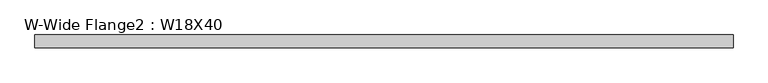
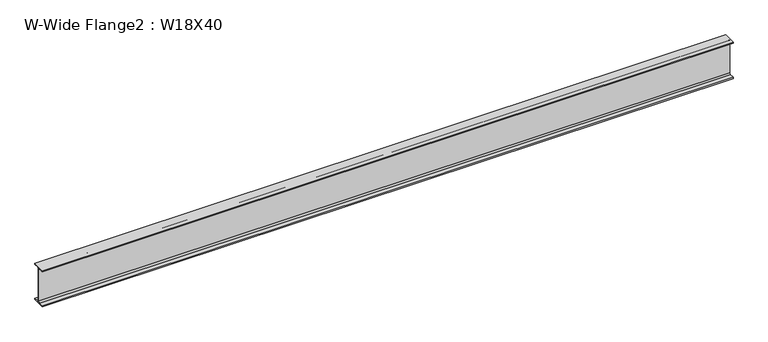
"""IFC4 building model written with IfcOpenShell, lengths in millimetres: beam geometry, W-Wide Flange2 : W18X40."""

import ifcopenshell
import ifcopenshell.guid

model = None  # the IFC model being written
_history = None  # IfcOwnerHistory: only IFC2X3 demands one
_inside = {}  # id of a spatial element -> (the spatial element, [elements in it])
_under = {}  # id of a project, library or spatial element -> (it, [spatial elements below it])
_declared = {}  # id of a project -> (the project, [libraries it declares])
_typed = {}  # id of a type object -> (the type object, [elements of that type])
_made_of = {}  # id of a material, layer set ... -> (it, [elements and type objects made of it])


def new_model(schema):
    """Start an empty IFC model of exactly this schema.

    Asked for "IFC4X3", IfcOpenShell would pick the latest addendum, in which some entities
    have other attributes; the version numbers below select the first issue.
    IFC2X3 requires an IfcOwnerHistory on every rooted entity: one is made here for all.
    """
    global model, _history
    if schema == "IFC4X3":
        model = ifcopenshell.file(schema_version=(4, 3, 0, 0))
    else:
        model = ifcopenshell.file(schema=schema)
    _inside.clear()
    _under.clear()
    _declared.clear()
    _typed.clear()
    _made_of.clear()
    _history = None
    if model.schema == "IFC2X3":
        org = make("IfcOrganization", Name="unknown")
        user = make(
            "IfcPersonAndOrganization",
            ThePerson=make("IfcPerson", FamilyName="unknown"),
            TheOrganization=org,
        )
        app = make(
            "IfcApplication",
            ApplicationDeveloper=org,
            Version="unknown",
            ApplicationFullName="unknown",
            ApplicationIdentifier="unknown",
        )
        _history = make(
            "IfcOwnerHistory",
            OwningUser=user,
            OwningApplication=app,
            ChangeAction="ADDED",
            CreationDate=0,
        )
    return model


def make(cls, **values):
    """One entity of the class cls with the attributes given. An attribute that is None is left unset."""
    return model.create_entity(
        cls, **{name: value for name, value in values.items() if value is not None}
    )


def rooted(cls, **values):
    """An entity with a GlobalId (a new one), such as an element, a storey or a relation."""
    return make(cls, GlobalId=ifcopenshell.guid.new(), OwnerHistory=_history, **values)


def si_unit(unit_type, name, prefix=None):
    """IfcSIUnit, for example si_unit("LENGTHUNIT", "METRE", prefix="MILLI")."""
    return make("IfcSIUnit", UnitType=unit_type, Prefix=prefix, Name=name)


def assignment(units):
    """IfcUnitAssignment: the units of a project."""
    return None if units is None else make("IfcUnitAssignment", Units=units)


def point(xyz):
    """IfcCartesianPoint."""
    return None if xyz is None else make("IfcCartesianPoint", Coordinates=xyz)


def direction(xyz):
    """IfcDirection."""
    return None if xyz is None else make("IfcDirection", DirectionRatios=xyz)


def frame(location, z_axis=None, x_axis=None):
    """IfcAxis2Placement3D, a coordinate frame: its origin and axes. An axis left out is left unset."""
    return make(
        "IfcAxis2Placement3D",
        Location=point(location),
        Axis=direction(z_axis),
        RefDirection=direction(x_axis),
    )


def frame_2d(location, x_axis=None):
    """IfcAxis2Placement2D, a coordinate frame in the plane: its origin and x axis."""
    return make(
        "IfcAxis2Placement2D", Location=point(location), RefDirection=direction(x_axis)
    )


def origin():
    """The frame at (0, 0, 0) with its axes left unset."""
    return frame((0.0, 0.0, 0.0))


def place(relative_to, where):
    """IfcLocalPlacement: puts the frame where relative to a parent placement (None: the world)."""
    return make(
        "IfcLocalPlacement", PlacementRelTo=relative_to, RelativePlacement=where
    )


def context(
    kind, dimensions, precision=None, world=None, true_north=None, identifier=None
):
    """IfcGeometricRepresentationContext, for example the 3D "Model" context."""
    return make(
        "IfcGeometricRepresentationContext",
        ContextIdentifier=identifier,
        ContextType=kind,
        CoordinateSpaceDimension=dimensions,
        Precision=precision,
        WorldCoordinateSystem=world,
        TrueNorth=true_north,
    )


def project(units=None, contexts=None):
    """IfcProject with its units and contexts."""
    return rooted(
        "IfcProject",
        Name="project",
        RepresentationContexts=contexts,
        UnitsInContext=assignment(units),
    )


def spatial(cls, under=None, at=None, **own):
    """A site, building, storey or space (cls), placed at a placement, below another one or the project."""
    s = rooted(cls, ObjectPlacement=at, **own)
    if under is not None:
        _under.setdefault(under.id(), (under, []))[1].append(s)
    return s


def polyline(points):
    """IfcPolyline through the points."""
    return make("IfcPolyline", Points=[point(p) for p in points])


def circle_curve(where, radius):
    """IfcCircle in the frame where."""
    return make("IfcCircle", Position=where, Radius=radius)


def trimmed(basis, trim1, trim2, sense, master):
    """IfcTrimmedCurve: the piece of a basis curve between two trims."""
    return make(
        "IfcTrimmedCurve",
        BasisCurve=basis,
        Trim1=trim1,
        Trim2=trim2,
        SenseAgreement=sense,
        MasterRepresentation=master,
    )


def segment(curve, same_sense, transition):
    """IfcCompositeCurveSegment."""
    return make(
        "IfcCompositeCurveSegment",
        Transition=transition,
        SameSense=same_sense,
        ParentCurve=curve,
    )


def composite_curve(segments, self_intersect=None):
    """IfcCompositeCurve: segments joined end to end."""
    return make("IfcCompositeCurve", Segments=segments, SelfIntersect=self_intersect)


def outline(outer, holes=None, kind="AREA"):
    """IfcArbitraryClosedProfileDef: a profile drawn as a closed curve; with holes, ...WithVoids."""
    if holes is None:
        return make("IfcArbitraryClosedProfileDef", ProfileType=kind, OuterCurve=outer)
    return make(
        "IfcArbitraryProfileDefWithVoids",
        ProfileType=kind,
        OuterCurve=outer,
        InnerCurves=holes,
    )


def extrude(swept, where, along, depth):
    """IfcExtrudedAreaSolid: the profile swept, set in the frame where, extruded along a direction by depth."""
    return make(
        "IfcExtrudedAreaSolid",
        SweptArea=swept,
        Position=where,
        ExtrudedDirection=direction(along),
        Depth=depth,
    )


def shape(context_of_items, identifier, shape_type, items):
    """IfcShapeRepresentation: the items that make up one representation, for example the "Body"."""
    return make(
        "IfcShapeRepresentation",
        ContextOfItems=context_of_items,
        RepresentationIdentifier=identifier,
        RepresentationType=shape_type,
        Items=items,
    )


def source(mapping_origin, context_of_items, identifier, shape_type, items):
    """IfcRepresentationMap: a shape defined once, which mapped items show again and again."""
    return make(
        "IfcRepresentationMap",
        MappingOrigin=mapping_origin,
        MappedRepresentation=shape(context_of_items, identifier, shape_type, items),
    )


def transform(
    local_origin,
    x_axis=None,
    y_axis=None,
    z_axis=None,
    scale=None,
    scale2=None,
    scale3=None,
    uniform=True,
):
    """IfcCartesianTransformationOperator3D, or its non-uniform kind. x_axis, y_axis, z_axis: its Axis1, 2, 3."""
    if uniform:
        return make(
            "IfcCartesianTransformationOperator3D",
            Axis1=direction(x_axis),
            Axis2=direction(y_axis),
            LocalOrigin=point(local_origin),
            Scale=scale,
            Axis3=direction(z_axis),
        )
    return make(
        "IfcCartesianTransformationOperator3DnonUniform",
        Axis1=direction(x_axis),
        Axis2=direction(y_axis),
        LocalOrigin=point(local_origin),
        Scale=scale,
        Axis3=direction(z_axis),
        Scale2=scale2,
        Scale3=scale3,
    )


def mapped(mapping_source, mapping_target):
    """IfcMappedItem: shows the shape of a source again, moved by a transform."""
    return make(
        "IfcMappedItem", MappingSource=mapping_source, MappingTarget=mapping_target
    )


def made_of(thing, what):
    """Note that an element or type object is made of a material, layer set ...; save() writes the relation."""
    if what is not None:
        _made_of.setdefault(what.id(), (what, []))[1].append(thing)
    return thing


def element(
    cls,
    number,
    at=None,
    inside=None,
    cuts=None,
    type_object=None,
    material=None,
    context=None,
    identifier="Body",
    shape_type=None,
    held_by="IfcProductDefinitionShape",
    body=None,
    shapes=None,
    **own,
):
    """One element of the class cls, such as IfcWall. Its Tag is "e" and its number.

    at: its placement. inside: the storey or other place that contains it. cuts: it is an
    opening in that element (IfcRelVoidsElement). A single representation is given by context,
    identifier, shape_type and body (its items); several are given by shapes. held_by: the class
    of the entity that holds the representations. save() writes the other relations.
    """
    e = rooted(cls, Tag="e%d" % number, ObjectPlacement=at, **own)
    if body is not None:
        shapes = [shape(context, identifier, shape_type, body)]
    if shapes is not None:
        e.Representation = make(held_by, Representations=shapes)
    if inside is not None:
        _inside.setdefault(inside.id(), (inside, []))[1].append(e)
    if cuts is not None:
        rooted(
            "IfcRelVoidsElement", RelatingBuildingElement=cuts, RelatedOpeningElement=e
        )
    if type_object is not None:
        _typed.setdefault(type_object.id(), (type_object, []))[1].append(e)
    return made_of(e, material)


def aggregate(whole, parts):
    """IfcRelAggregates: a whole, such as a stair, and the parts it consists of."""
    return rooted("IfcRelAggregates", RelatingObject=whole, RelatedObjects=parts)


def save(model, path):
    """Write the relations noted so far, then the file.

    IfcRelAggregates (storeys below a building ...), IfcRelContainedInSpatialStructure (elements
    in a storey), IfcRelDefinesByType, IfcRelAssociatesMaterial and IfcRelDeclares: one each for
    every whole, place, type object, material and project.
    """
    for whole, parts in _under.values():
        aggregate(whole, parts)
    for where, things in _inside.values():
        rooted(
            "IfcRelContainedInSpatialStructure",
            RelatedElements=things,
            RelatingStructure=where,
        )
    for kind, things in _typed.values():
        rooted("IfcRelDefinesByType", RelatedObjects=things, RelatingType=kind)
    for what, things in _made_of.values():
        rooted("IfcRelAssociatesMaterial", RelatedObjects=things, RelatingMaterial=what)
    for by, libraries in _declared.values():
        rooted("IfcRelDeclares", RelatingContext=by, RelatedDefinitions=libraries)
    model.write(path)


def w_wide_flange2_w18x40_2ea4b68e(model_context):
    return source(origin(), model_context, "Body", "SweptSolid", [
        extrude(outline(composite_curve([segment(polyline([(76.454, -213.995), (76.454, -227.33), (-76.454, -227.33), (-76.454, -213.995), (-20.828, -213.995)]), True, "CONTINUOUS"), segment(trimmed(circle_curve(frame_2d((-20.828, -197.1675)), 16.8275), [point((-20.828, -213.995))], [point((-4.0005, -197.1675))], True, "CARTESIAN"), True, "CONTINUOUS"), segment(polyline([(-4.0005, -197.1675), (-4.0005, 197.1675)]), True, "CONTINUOUS"), segment(trimmed(circle_curve(frame_2d((-20.828, 197.1675)), 16.8275), [point((-4.0005, 197.1675))], [point((-20.828, 213.995))], True, "CARTESIAN"), True, "CONTINUOUS"), segment(polyline([(-20.828, 213.995), (-76.454, 213.995), (-76.454, 227.33), (76.454, 227.33), (76.454, 213.995), (20.828, 213.995)]), True, "CONTINUOUS"), segment(trimmed(circle_curve(frame_2d((20.828, 197.1675)), 16.8275), [point((20.828, 213.995))], [point((4.0005, 197.1675))], True, "CARTESIAN"), True, "CONTINUOUS"), segment(polyline([(4.0005, 197.1675), (4.0005, -197.1675)]), True, "CONTINUOUS"), segment(trimmed(circle_curve(frame_2d((20.828, -197.1675)), 16.8275), [point((4.0005, -197.1675))], [point((20.828, -213.995))], True, "CARTESIAN"), True, "CONTINUOUS"), segment(polyline([(20.828, -213.995), (76.454, -213.995)]), True, "CONTINUOUS")], self_intersect=False)), frame((-4100.5125, 0.0, 0.0), z_axis=(1.0, 0.0, 0.0), x_axis=(0.0, 1.0, 0.0)), (0.0, 0.0, 1.0), 8201.025),
    ])


if __name__ == "__main__":
    model = new_model("IFC4")
    model_context = context("Model", 3, world=origin())
    ifc_project = project(units=[si_unit("LENGTHUNIT", "METRE", prefix="MILLI")], contexts=[model_context])
    site = spatial("IfcSite", under=ifc_project)
    building = spatial("IfcBuilding", under=site)
    placement = place(None, origin())
    w_wide_flange2_w18x40_shape = w_wide_flange2_w18x40_2ea4b68e(model_context)
    element("IfcBeam", 1, ObjectType="W-Wide Flange2 : W18X40", at=placement, inside=building, context=model_context, shape_type="MappedRepresentation", body=[
        mapped(w_wide_flange2_w18x40_shape, transform((0.0, 0.0, 0.0), x_axis=(1.0, 0.0, 0.0), y_axis=(0.0, 1.0, 0.0), z_axis=(0.0, 0.0, 1.0))),
    ])
    save(model, "model.ifc")

# Revit data of these elements
# Type "W-Wide Flange2 : W18X40"
#   Assembly Code = "B10"
#   W = 40
#   Length [instance default] = 5' - 0"
#   bf = 0' - 6.02"
#   d = 1' - 5.9"
#   k = 0' - 1 3/16"
#   k2 = 0' - 0.6625"
#   tf = 0' - 0.525"
#   tw = 0' - 0.315"
#   A = 0.0819444 SF
#   Structural Material [instance default] = Steel ASTM A992
# Element 1 (IfcBeam, "W-Wide Flange2 : W18X40")
#   Materials on its faces: "Steel ASTM A992"
# Materials
#   "Steel ASTM A992": class "Metal", colour RGB 199 199 199, transparency 0, Description = "Structural steel 50ksi", Cost = 0
